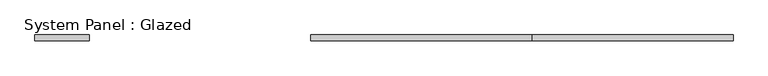
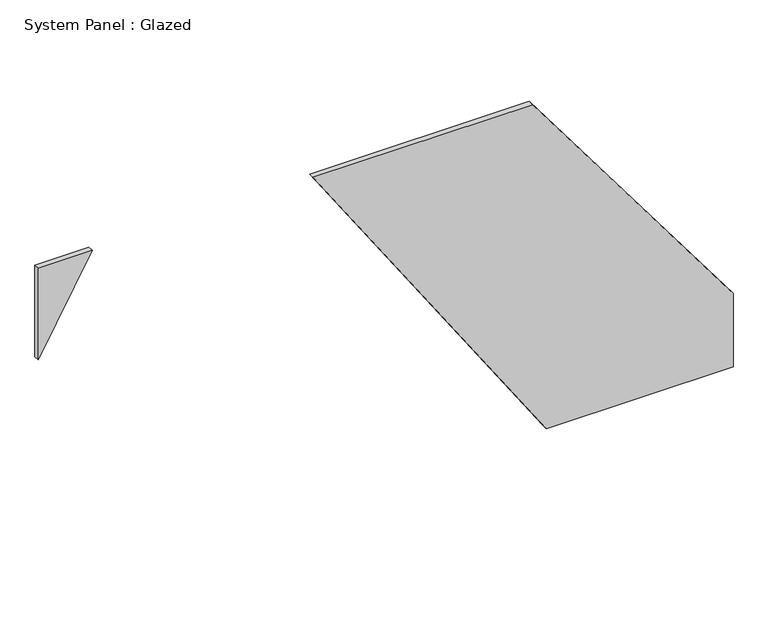
"""IFC4 building model written with IfcOpenShell, lengths in millimetres: plate geometry, System Panel : Glazed."""

from ifc_helpers import new_model, si_unit, frame, origin, place, context, project, spatial, polyline, outline, extrude, source, transform, mapped, element, save


def system_panel_glazed_40b087d6(model_context):
    return source(origin(), model_context, "Body", "SweptSolid", [
        extrude(outline(polyline([(0.0, 692.8059979), (0.0, 1500.0), (335.4842192, 1500.0), (1500.0, 634.4904554), (1500.0, -314.0552731), (0.0, 692.8059979)])), frame((0.0, 24.5, 0.0), z_axis=(0.0, 1.0, 0.0), x_axis=(0.0, 0.0, 1.0)), (0.0, 0.0, 1.0), 25.0),
        extrude(outline(polyline([(1500.0, -1500.0), (1081.9101827, -1500.0), (1500.0, -1267.018144), (1500.0, -1500.0)])), frame((0.0, 24.5, 0.0), z_axis=(0.0, 1.0, 0.0), x_axis=(0.0, 0.0, 1.0)), (0.0, 0.0, 1.0), 25.0),
    ])


if __name__ == "__main__":
    model = new_model("IFC4")
    model_context = context("Model", 3, world=origin())
    ifc_project = project(units=[si_unit("LENGTHUNIT", "METRE", prefix="MILLI")], contexts=[model_context])
    site = spatial("IfcSite", under=ifc_project)
    building = spatial("IfcBuilding", under=site)
    placement = place(None, origin())
    system_panel_glazed_shape = system_panel_glazed_40b087d6(model_context)
    element("IfcPlate", 1, ObjectType="System Panel : Glazed", at=placement, inside=building, context=model_context, shape_type="MappedRepresentation", body=[
        mapped(system_panel_glazed_shape, transform((0.0, 0.0, 0.0), x_axis=(1.0, 0.0, 0.0), y_axis=(0.0, 1.0, 0.0), z_axis=(0.0, 0.0, 1.0))),
    ])
    save(model, "model.ifc")

# Revit data of these elements
# Type "System Panel : Glazed"
#   Construction Type Id = "GSP4R"
#   Analytic Construction = "1/8 in Pilkington single glazing"
#   Visual Light Transmittance = 0.9
#   Solar Heat Gain Coefficient = 0.86
#   Heat Transfer Coefficient (U) = 6.7069 W/(m²·K)
#   Define Thermal Properties by = 1
# Element 1 (IfcPlate, "System Panel : Glazed")
#   Materials on its faces: "Glass"
# Materials
#   "Glass": class "Glass", colour RGB 0 128 192, transparency 0.9, Description = "Soda Lime Glass", Cost = 0
